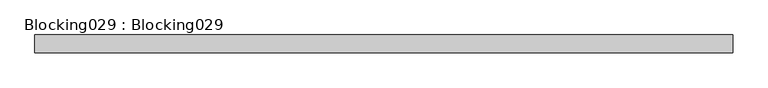
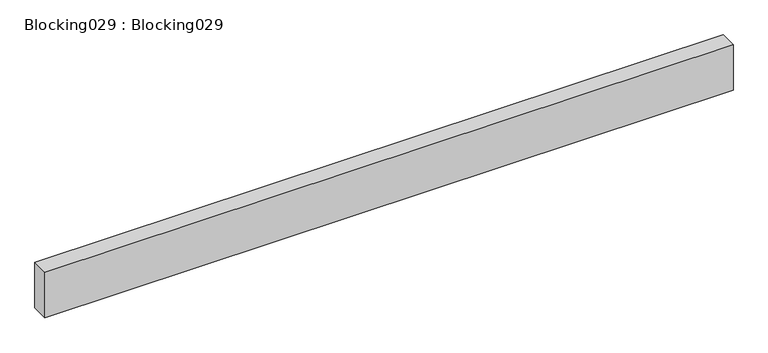
"""IFC4 building model written with IfcOpenShell, lengths in millimetres: proxy geometry, Blocking029 : Blocking029."""

from ifc_helpers import new_model, si_unit, frame, origin, place, context, project, spatial, polyline, outline, extrude, source, transform, mapped, element, save


def blocking029_blocking029_4256e288(model_context):
    return source(origin(), model_context, "Body", "SweptSolid", [
        extrude(outline(polyline([(14383.0178845, -4586.7425368), (14383.0178845, -4637.5425368), (12383.0178845, -4637.5425368), (12383.0178845, -4586.7425368), (14383.0178845, -4586.7425368)])), frame((0.0, 0.0, 39019.0959974), z_axis=(0.0, 0.0, 1.0), x_axis=(1.0, 0.0, 0.0)), (0.0, 0.0, 1.0), 139.7),
    ])


if __name__ == "__main__":
    model = new_model("IFC4")
    model_context = context("Model", 3, world=origin())
    ifc_project = project(units=[si_unit("LENGTHUNIT", "METRE", prefix="MILLI")], contexts=[model_context])
    site = spatial("IfcSite", under=ifc_project)
    building = spatial("IfcBuilding", under=site)
    placement = place(None, origin())
    blocking029_blocking029_shape = blocking029_blocking029_4256e288(model_context)
    element("IfcBuildingElementProxy", 1, Name="Blocking029 : Blocking029", ObjectType="Blocking029 : Blocking029", at=placement, inside=building, context=model_context, shape_type="MappedRepresentation", body=[
        mapped(blocking029_blocking029_shape, transform((0.0, 0.0, 0.0), x_axis=(1.0, 0.0, 0.0), y_axis=(0.0, 1.0, 0.0), z_axis=(0.0, 0.0, 1.0))),
    ])
    save(model, "model.ifc")

# Revit data of these elements
# Type "Blocking029 : Blocking029"
#   NameOverride = "Blocking029"
# Element 1 (IfcBuildingElementProxy, "Blocking029 : Blocking029")
#   Materials on its faces: "WOOD BLOCKING AS REQUIRED"
# Materials
#   "WOOD BLOCKING AS REQUIRED": class "Unassigned", colour RGB 166 124 85, transparency 0, Cost = 0
